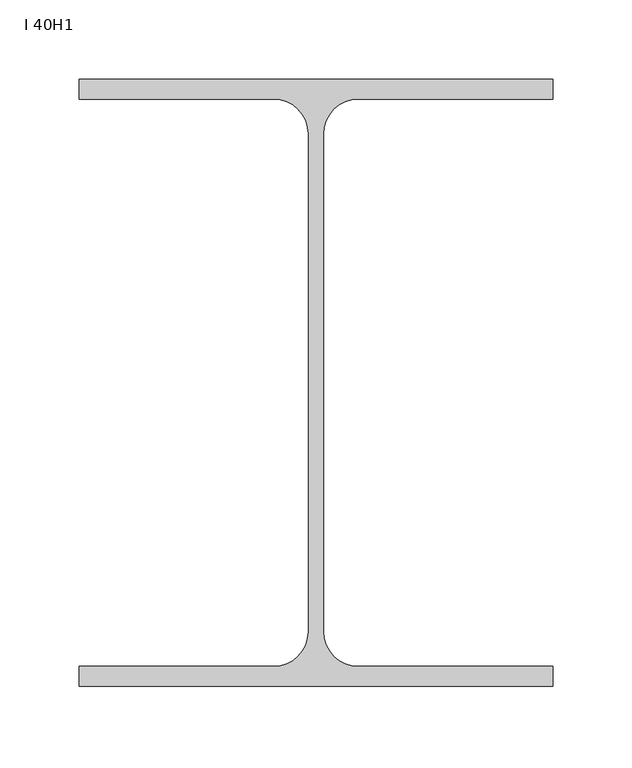
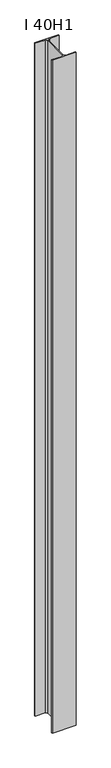
"""IFC4 building model written with IfcOpenShell, lengths in millimetres: column geometry, Двутавровая балка с широкими полками (ASTO20-93)-Колонна : I 40H1."""

import ifcopenshell
import ifcopenshell.guid

model = None  # the IFC model being written
_history = None  # IfcOwnerHistory: only IFC2X3 demands one
_inside = {}  # id of a spatial element -> (the spatial element, [elements in it])
_under = {}  # id of a project, library or spatial element -> (it, [spatial elements below it])
_declared = {}  # id of a project -> (the project, [libraries it declares])
_typed = {}  # id of a type object -> (the type object, [elements of that type])
_made_of = {}  # id of a material, layer set ... -> (it, [elements and type objects made of it])


def new_model(schema):
    """Start an empty IFC model of exactly this schema.

    Asked for "IFC4X3", IfcOpenShell would pick the latest addendum, in which some entities
    have other attributes; the version numbers below select the first issue.
    IFC2X3 requires an IfcOwnerHistory on every rooted entity: one is made here for all.
    """
    global model, _history
    if schema == "IFC4X3":
        model = ifcopenshell.file(schema_version=(4, 3, 0, 0))
    else:
        model = ifcopenshell.file(schema=schema)
    _inside.clear()
    _under.clear()
    _declared.clear()
    _typed.clear()
    _made_of.clear()
    _history = None
    if model.schema == "IFC2X3":
        org = make("IfcOrganization", Name="unknown")
        user = make(
            "IfcPersonAndOrganization",
            ThePerson=make("IfcPerson", FamilyName="unknown"),
            TheOrganization=org,
        )
        app = make(
            "IfcApplication",
            ApplicationDeveloper=org,
            Version="unknown",
            ApplicationFullName="unknown",
            ApplicationIdentifier="unknown",
        )
        _history = make(
            "IfcOwnerHistory",
            OwningUser=user,
            OwningApplication=app,
            ChangeAction="ADDED",
            CreationDate=0,
        )
    return model


def make(cls, **values):
    """One entity of the class cls with the attributes given. An attribute that is None is left unset."""
    return model.create_entity(
        cls, **{name: value for name, value in values.items() if value is not None}
    )


def rooted(cls, **values):
    """An entity with a GlobalId (a new one), such as an element, a storey or a relation."""
    return make(cls, GlobalId=ifcopenshell.guid.new(), OwnerHistory=_history, **values)


def si_unit(unit_type, name, prefix=None):
    """IfcSIUnit, for example si_unit("LENGTHUNIT", "METRE", prefix="MILLI")."""
    return make("IfcSIUnit", UnitType=unit_type, Prefix=prefix, Name=name)


def assignment(units):
    """IfcUnitAssignment: the units of a project."""
    return None if units is None else make("IfcUnitAssignment", Units=units)


def point(xyz):
    """IfcCartesianPoint."""
    return None if xyz is None else make("IfcCartesianPoint", Coordinates=xyz)


def direction(xyz):
    """IfcDirection."""
    return None if xyz is None else make("IfcDirection", DirectionRatios=xyz)


def frame(location, z_axis=None, x_axis=None):
    """IfcAxis2Placement3D, a coordinate frame: its origin and axes. An axis left out is left unset."""
    return make(
        "IfcAxis2Placement3D",
        Location=point(location),
        Axis=direction(z_axis),
        RefDirection=direction(x_axis),
    )


def frame_2d(location, x_axis=None):
    """IfcAxis2Placement2D, a coordinate frame in the plane: its origin and x axis."""
    return make(
        "IfcAxis2Placement2D", Location=point(location), RefDirection=direction(x_axis)
    )


def origin():
    """The frame at (0, 0, 0) with its axes left unset."""
    return frame((0.0, 0.0, 0.0))


def origin_with_axes():
    """The frame at (0, 0, 0) with the z axis (0, 0, 1) and the x axis (1, 0, 0) written out."""
    return frame((0.0, 0.0, 0.0), z_axis=(0.0, 0.0, 1.0), x_axis=(1.0, 0.0, 0.0))


def place(relative_to, where):
    """IfcLocalPlacement: puts the frame where relative to a parent placement (None: the world)."""
    return make(
        "IfcLocalPlacement", PlacementRelTo=relative_to, RelativePlacement=where
    )


def context(
    kind, dimensions, precision=None, world=None, true_north=None, identifier=None
):
    """IfcGeometricRepresentationContext, for example the 3D "Model" context."""
    return make(
        "IfcGeometricRepresentationContext",
        ContextIdentifier=identifier,
        ContextType=kind,
        CoordinateSpaceDimension=dimensions,
        Precision=precision,
        WorldCoordinateSystem=world,
        TrueNorth=true_north,
    )


def project(units=None, contexts=None):
    """IfcProject with its units and contexts."""
    return rooted(
        "IfcProject",
        Name="project",
        RepresentationContexts=contexts,
        UnitsInContext=assignment(units),
    )


def spatial(cls, under=None, at=None, **own):
    """A site, building, storey or space (cls), placed at a placement, below another one or the project."""
    s = rooted(cls, ObjectPlacement=at, **own)
    if under is not None:
        _under.setdefault(under.id(), (under, []))[1].append(s)
    return s


def polyline(points):
    """IfcPolyline through the points."""
    return make("IfcPolyline", Points=[point(p) for p in points])


def circle_curve(where, radius):
    """IfcCircle in the frame where."""
    return make("IfcCircle", Position=where, Radius=radius)


def trimmed(basis, trim1, trim2, sense, master):
    """IfcTrimmedCurve: the piece of a basis curve between two trims."""
    return make(
        "IfcTrimmedCurve",
        BasisCurve=basis,
        Trim1=trim1,
        Trim2=trim2,
        SenseAgreement=sense,
        MasterRepresentation=master,
    )


def segment(curve, same_sense, transition):
    """IfcCompositeCurveSegment."""
    return make(
        "IfcCompositeCurveSegment",
        Transition=transition,
        SameSense=same_sense,
        ParentCurve=curve,
    )


def composite_curve(segments, self_intersect=None):
    """IfcCompositeCurve: segments joined end to end."""
    return make("IfcCompositeCurve", Segments=segments, SelfIntersect=self_intersect)


def outline(outer, holes=None, kind="AREA"):
    """IfcArbitraryClosedProfileDef: a profile drawn as a closed curve; with holes, ...WithVoids."""
    if holes is None:
        return make("IfcArbitraryClosedProfileDef", ProfileType=kind, OuterCurve=outer)
    return make(
        "IfcArbitraryProfileDefWithVoids",
        ProfileType=kind,
        OuterCurve=outer,
        InnerCurves=holes,
    )


def extrude(swept, where, along, depth):
    """IfcExtrudedAreaSolid: the profile swept, set in the frame where, extruded along a direction by depth."""
    return make(
        "IfcExtrudedAreaSolid",
        SweptArea=swept,
        Position=where,
        ExtrudedDirection=direction(along),
        Depth=depth,
    )


def shape(context_of_items, identifier, shape_type, items):
    """IfcShapeRepresentation: the items that make up one representation, for example the "Body"."""
    return make(
        "IfcShapeRepresentation",
        ContextOfItems=context_of_items,
        RepresentationIdentifier=identifier,
        RepresentationType=shape_type,
        Items=items,
    )


def source(mapping_origin, context_of_items, identifier, shape_type, items):
    """IfcRepresentationMap: a shape defined once, which mapped items show again and again."""
    return make(
        "IfcRepresentationMap",
        MappingOrigin=mapping_origin,
        MappedRepresentation=shape(context_of_items, identifier, shape_type, items),
    )


def transform(
    local_origin,
    x_axis=None,
    y_axis=None,
    z_axis=None,
    scale=None,
    scale2=None,
    scale3=None,
    uniform=True,
):
    """IfcCartesianTransformationOperator3D, or its non-uniform kind. x_axis, y_axis, z_axis: its Axis1, 2, 3."""
    if uniform:
        return make(
            "IfcCartesianTransformationOperator3D",
            Axis1=direction(x_axis),
            Axis2=direction(y_axis),
            LocalOrigin=point(local_origin),
            Scale=scale,
            Axis3=direction(z_axis),
        )
    return make(
        "IfcCartesianTransformationOperator3DnonUniform",
        Axis1=direction(x_axis),
        Axis2=direction(y_axis),
        LocalOrigin=point(local_origin),
        Scale=scale,
        Axis3=direction(z_axis),
        Scale2=scale2,
        Scale3=scale3,
    )


def mapped(mapping_source, mapping_target):
    """IfcMappedItem: shows the shape of a source again, moved by a transform."""
    return make(
        "IfcMappedItem", MappingSource=mapping_source, MappingTarget=mapping_target
    )


def made_of(thing, what):
    """Note that an element or type object is made of a material, layer set ...; save() writes the relation."""
    if what is not None:
        _made_of.setdefault(what.id(), (what, []))[1].append(thing)
    return thing


def element(
    cls,
    number,
    at=None,
    inside=None,
    cuts=None,
    type_object=None,
    material=None,
    context=None,
    identifier="Body",
    shape_type=None,
    held_by="IfcProductDefinitionShape",
    body=None,
    shapes=None,
    **own,
):
    """One element of the class cls, such as IfcWall. Its Tag is "e" and its number.

    at: its placement. inside: the storey or other place that contains it. cuts: it is an
    opening in that element (IfcRelVoidsElement). A single representation is given by context,
    identifier, shape_type and body (its items); several are given by shapes. held_by: the class
    of the entity that holds the representations. save() writes the other relations.
    """
    e = rooted(cls, Tag="e%d" % number, ObjectPlacement=at, **own)
    if body is not None:
        shapes = [shape(context, identifier, shape_type, body)]
    if shapes is not None:
        e.Representation = make(held_by, Representations=shapes)
    if inside is not None:
        _inside.setdefault(inside.id(), (inside, []))[1].append(e)
    if cuts is not None:
        rooted(
            "IfcRelVoidsElement", RelatingBuildingElement=cuts, RelatedOpeningElement=e
        )
    if type_object is not None:
        _typed.setdefault(type_object.id(), (type_object, []))[1].append(e)
    return made_of(e, material)


def aggregate(whole, parts):
    """IfcRelAggregates: a whole, such as a stair, and the parts it consists of."""
    return rooted("IfcRelAggregates", RelatingObject=whole, RelatedObjects=parts)


def save(model, path):
    """Write the relations noted so far, then the file.

    IfcRelAggregates (storeys below a building ...), IfcRelContainedInSpatialStructure (elements
    in a storey), IfcRelDefinesByType, IfcRelAssociatesMaterial and IfcRelDeclares: one each for
    every whole, place, type object, material and project.
    """
    for whole, parts in _under.values():
        aggregate(whole, parts)
    for where, things in _inside.values():
        rooted(
            "IfcRelContainedInSpatialStructure",
            RelatedElements=things,
            RelatingStructure=where,
        )
    for kind, things in _typed.values():
        rooted("IfcRelDefinesByType", RelatedObjects=things, RelatingType=kind)
    for what, things in _made_of.values():
        rooted("IfcRelAssociatesMaterial", RelatedObjects=things, RelatingMaterial=what)
    for by, libraries in _declared.values():
        rooted("IfcRelDeclares", RelatingContext=by, RelatedDefinitions=libraries)
    model.write(path)


def i_40h1_edde52e3(model_context):
    return source(origin(), model_context, "Body", "SweptSolid", [
        extrude(outline(composite_curve([segment(polyline([(-149.5, -178.5), (-26.75, -178.5)]), True, "CONTINUOUS"), segment(trimmed(circle_curve(frame_2d((-26.75, -156.5)), 22.0), [point((-26.75, -178.5))], [point((-4.75, -156.5))], True, "CARTESIAN"), True, "CONTINUOUS"), segment(polyline([(-4.75, -156.5), (-4.75, 157.5)]), True, "CONTINUOUS"), segment(trimmed(circle_curve(frame_2d((-26.75, 157.5)), 22.0), [point((-4.75, 157.5))], [point((-26.75, 179.5))], True, "CARTESIAN"), True, "CONTINUOUS"), segment(polyline([(-26.75, 179.5), (-149.5, 179.5), (-149.5, 192.0), (149.5, 192.0), (149.5, 179.5), (26.75, 179.5)]), True, "CONTINUOUS"), segment(trimmed(circle_curve(frame_2d((26.75, 157.5)), 22.0), [point((26.75, 179.5))], [point((4.75, 157.5))], True, "CARTESIAN"), True, "CONTINUOUS"), segment(polyline([(4.75, 157.5), (4.75, -156.5)]), True, "CONTINUOUS"), segment(trimmed(circle_curve(frame_2d((26.75, -156.5)), 22.0), [point((4.75, -156.5))], [point((26.75, -178.5))], True, "CARTESIAN"), True, "CONTINUOUS"), segment(polyline([(26.75, -178.5), (149.5, -178.5), (149.5, -191.0), (-149.5, -191.0), (-149.5, -178.5)]), True, "CONTINUOUS")], self_intersect=False)), origin_with_axes(), (0.0, 0.0, 1.0), 8923.3858447),
    ])


if __name__ == "__main__":
    model = new_model("IFC4")
    model_context = context("Model", 3, world=origin())
    ifc_project = project(units=[si_unit("LENGTHUNIT", "METRE", prefix="MILLI")], contexts=[model_context])
    site = spatial("IfcSite", under=ifc_project)
    building = spatial("IfcBuilding", under=site)
    placement = place(None, origin())
    i_40h1_shape = i_40h1_edde52e3(model_context)
    element("IfcColumn", 1, ObjectType="Двутавровая балка с широкими полками (ASTO20-93)-Колонна : I 40H1", at=placement, inside=building, context=model_context, shape_type="MappedRepresentation", body=[
        mapped(i_40h1_shape, transform((0.0, 0.0, 0.0), x_axis=(1.0, 0.0, 0.0), y_axis=(0.0, 1.0, 0.0), z_axis=(0.0, 0.0, 1.0))),
    ])
    save(model, "model.ifc")

# Revit data of these elements
# Type "Двутавровая балка с широкими полками (ASTO20-93)-Колонна : I 40H1"
#   ra = 22 mm
#   W = 0.868869
#   Vz = 191.5 mm
#   Vy = 149.5 mm
#   Vpz = 191.5 mm
#   Vpy = 149.5 mm
#   bf = 299 mm
#   d = 383 mm
#   tf = 12.5 mm
#   tw = 9.5 mm
#   A = 0.011291 m²
#   Structural Material [instance default] = Металл - Сталь - 345 МПa
#   Assembly Code = ""
# Element 1 (IfcColumn, "Двутавровая балка с широкими полками (ASTO20-93)-Колонна : I 40H1")
#   Structural Material = C345
#   Materials on its faces: "C345"
# Materials
#   "Металл - Сталь - 345 МПa": class "Металл", colour RGB 247 247 247, transparency 0
#   "C345": class "Не назначено", colour RGB 0 0 0, transparency 0
